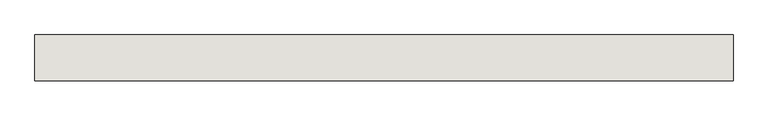
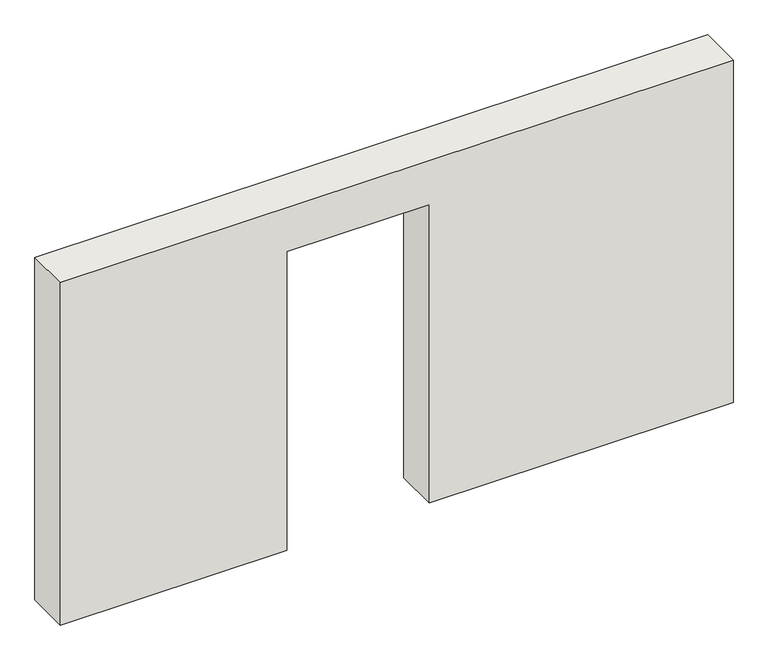
"""IFC4 building model written with IfcOpenShell, lengths in millimetres: wall geometry, 0_3d_modell."""

import ifcopenshell
import ifcopenshell.guid

model = None  # the IFC model being written
_history = None  # IfcOwnerHistory: only IFC2X3 demands one
_inside = {}  # id of a spatial element -> (the spatial element, [elements in it])
_under = {}  # id of a project, library or spatial element -> (it, [spatial elements below it])
_declared = {}  # id of a project -> (the project, [libraries it declares])
_typed = {}  # id of a type object -> (the type object, [elements of that type])
_made_of = {}  # id of a material, layer set ... -> (it, [elements and type objects made of it])


def new_model(schema):
    """Start an empty IFC model of exactly this schema.

    Asked for "IFC4X3", IfcOpenShell would pick the latest addendum, in which some entities
    have other attributes; the version numbers below select the first issue.
    IFC2X3 requires an IfcOwnerHistory on every rooted entity: one is made here for all.
    """
    global model, _history
    if schema == "IFC4X3":
        model = ifcopenshell.file(schema_version=(4, 3, 0, 0))
    else:
        model = ifcopenshell.file(schema=schema)
    _inside.clear()
    _under.clear()
    _declared.clear()
    _typed.clear()
    _made_of.clear()
    _history = None
    if model.schema == "IFC2X3":
        org = make("IfcOrganization", Name="unknown")
        user = make(
            "IfcPersonAndOrganization",
            ThePerson=make("IfcPerson", FamilyName="unknown"),
            TheOrganization=org,
        )
        app = make(
            "IfcApplication",
            ApplicationDeveloper=org,
            Version="unknown",
            ApplicationFullName="unknown",
            ApplicationIdentifier="unknown",
        )
        _history = make(
            "IfcOwnerHistory",
            OwningUser=user,
            OwningApplication=app,
            ChangeAction="ADDED",
            CreationDate=0,
        )
    return model


def make(cls, **values):
    """One entity of the class cls with the attributes given. An attribute that is None is left unset."""
    return model.create_entity(
        cls, **{name: value for name, value in values.items() if value is not None}
    )


def rooted(cls, **values):
    """An entity with a GlobalId (a new one), such as an element, a storey or a relation."""
    return make(cls, GlobalId=ifcopenshell.guid.new(), OwnerHistory=_history, **values)


def si_unit(unit_type, name, prefix=None):
    """IfcSIUnit, for example si_unit("LENGTHUNIT", "METRE", prefix="MILLI")."""
    return make("IfcSIUnit", UnitType=unit_type, Prefix=prefix, Name=name)


def assignment(units):
    """IfcUnitAssignment: the units of a project."""
    return None if units is None else make("IfcUnitAssignment", Units=units)


def point(xyz):
    """IfcCartesianPoint."""
    return None if xyz is None else make("IfcCartesianPoint", Coordinates=xyz)


def direction(xyz):
    """IfcDirection."""
    return None if xyz is None else make("IfcDirection", DirectionRatios=xyz)


def frame(location, z_axis=None, x_axis=None):
    """IfcAxis2Placement3D, a coordinate frame: its origin and axes. An axis left out is left unset."""
    return make(
        "IfcAxis2Placement3D",
        Location=point(location),
        Axis=direction(z_axis),
        RefDirection=direction(x_axis),
    )


def origin():
    """The frame at (0, 0, 0) with its axes left unset."""
    return frame((0.0, 0.0, 0.0))


def place(relative_to, where):
    """IfcLocalPlacement: puts the frame where relative to a parent placement (None: the world)."""
    return make(
        "IfcLocalPlacement", PlacementRelTo=relative_to, RelativePlacement=where
    )


def context(
    kind, dimensions, precision=None, world=None, true_north=None, identifier=None
):
    """IfcGeometricRepresentationContext, for example the 3D "Model" context."""
    return make(
        "IfcGeometricRepresentationContext",
        ContextIdentifier=identifier,
        ContextType=kind,
        CoordinateSpaceDimension=dimensions,
        Precision=precision,
        WorldCoordinateSystem=world,
        TrueNorth=true_north,
    )


def project(units=None, contexts=None):
    """IfcProject with its units and contexts."""
    return rooted(
        "IfcProject",
        Name="project",
        RepresentationContexts=contexts,
        UnitsInContext=assignment(units),
    )


def spatial(cls, under=None, at=None, **own):
    """A site, building, storey or space (cls), placed at a placement, below another one or the project."""
    s = rooted(cls, ObjectPlacement=at, **own)
    if under is not None:
        _under.setdefault(under.id(), (under, []))[1].append(s)
    return s


def polyline(points):
    """IfcPolyline through the points."""
    return make("IfcPolyline", Points=[point(p) for p in points])


def outline(outer, holes=None, kind="AREA"):
    """IfcArbitraryClosedProfileDef: a profile drawn as a closed curve; with holes, ...WithVoids."""
    if holes is None:
        return make("IfcArbitraryClosedProfileDef", ProfileType=kind, OuterCurve=outer)
    return make(
        "IfcArbitraryProfileDefWithVoids",
        ProfileType=kind,
        OuterCurve=outer,
        InnerCurves=holes,
    )


def extrude(swept, where, along, depth):
    """IfcExtrudedAreaSolid: the profile swept, set in the frame where, extruded along a direction by depth."""
    return make(
        "IfcExtrudedAreaSolid",
        SweptArea=swept,
        Position=where,
        ExtrudedDirection=direction(along),
        Depth=depth,
    )


def shape(context_of_items, identifier, shape_type, items):
    """IfcShapeRepresentation: the items that make up one representation, for example the "Body"."""
    return make(
        "IfcShapeRepresentation",
        ContextOfItems=context_of_items,
        RepresentationIdentifier=identifier,
        RepresentationType=shape_type,
        Items=items,
    )


def source(mapping_origin, context_of_items, identifier, shape_type, items):
    """IfcRepresentationMap: a shape defined once, which mapped items show again and again."""
    return make(
        "IfcRepresentationMap",
        MappingOrigin=mapping_origin,
        MappedRepresentation=shape(context_of_items, identifier, shape_type, items),
    )


def transform(
    local_origin,
    x_axis=None,
    y_axis=None,
    z_axis=None,
    scale=None,
    scale2=None,
    scale3=None,
    uniform=True,
):
    """IfcCartesianTransformationOperator3D, or its non-uniform kind. x_axis, y_axis, z_axis: its Axis1, 2, 3."""
    if uniform:
        return make(
            "IfcCartesianTransformationOperator3D",
            Axis1=direction(x_axis),
            Axis2=direction(y_axis),
            LocalOrigin=point(local_origin),
            Scale=scale,
            Axis3=direction(z_axis),
        )
    return make(
        "IfcCartesianTransformationOperator3DnonUniform",
        Axis1=direction(x_axis),
        Axis2=direction(y_axis),
        LocalOrigin=point(local_origin),
        Scale=scale,
        Axis3=direction(z_axis),
        Scale2=scale2,
        Scale3=scale3,
    )


def mapped(mapping_source, mapping_target):
    """IfcMappedItem: shows the shape of a source again, moved by a transform."""
    return make(
        "IfcMappedItem", MappingSource=mapping_source, MappingTarget=mapping_target
    )


def made_of(thing, what):
    """Note that an element or type object is made of a material, layer set ...; save() writes the relation."""
    if what is not None:
        _made_of.setdefault(what.id(), (what, []))[1].append(thing)
    return thing


def element(
    cls,
    number,
    at=None,
    inside=None,
    cuts=None,
    type_object=None,
    material=None,
    context=None,
    identifier="Body",
    shape_type=None,
    held_by="IfcProductDefinitionShape",
    body=None,
    shapes=None,
    **own,
):
    """One element of the class cls, such as IfcWall. Its Tag is "e" and its number.

    at: its placement. inside: the storey or other place that contains it. cuts: it is an
    opening in that element (IfcRelVoidsElement). A single representation is given by context,
    identifier, shape_type and body (its items); several are given by shapes. held_by: the class
    of the entity that holds the representations. save() writes the other relations.
    """
    e = rooted(cls, Tag="e%d" % number, ObjectPlacement=at, **own)
    if body is not None:
        shapes = [shape(context, identifier, shape_type, body)]
    if shapes is not None:
        e.Representation = make(held_by, Representations=shapes)
    if inside is not None:
        _inside.setdefault(inside.id(), (inside, []))[1].append(e)
    if cuts is not None:
        rooted(
            "IfcRelVoidsElement", RelatingBuildingElement=cuts, RelatedOpeningElement=e
        )
    if type_object is not None:
        _typed.setdefault(type_object.id(), (type_object, []))[1].append(e)
    return made_of(e, material)


def aggregate(whole, parts):
    """IfcRelAggregates: a whole, such as a stair, and the parts it consists of."""
    return rooted("IfcRelAggregates", RelatingObject=whole, RelatedObjects=parts)


def save(model, path):
    """Write the relations noted so far, then the file.

    IfcRelAggregates (storeys below a building ...), IfcRelContainedInSpatialStructure (elements
    in a storey), IfcRelDefinesByType, IfcRelAssociatesMaterial and IfcRelDeclares: one each for
    every whole, place, type object, material and project.
    """
    for whole, parts in _under.values():
        aggregate(whole, parts)
    for where, things in _inside.values():
        rooted(
            "IfcRelContainedInSpatialStructure",
            RelatedElements=things,
            RelatingStructure=where,
        )
    for kind, things in _typed.values():
        rooted("IfcRelDefinesByType", RelatedObjects=things, RelatingType=kind)
    for what, things in _made_of.values():
        rooted("IfcRelAssociatesMaterial", RelatedObjects=things, RelatingMaterial=what)
    for by, libraries in _declared.values():
        rooted("IfcRelDeclares", RelatingContext=by, RelatedDefinitions=libraries)
    model.write(path)


def wall_d88cb43b(model_context):
    return source(origin(), model_context, "Body", "SweptSolid", [
        extrude(outline(polyline([(2510.0, 2935.0), (0.0, 2935.0), (0.0, 5350.0), (2880.0, 5350.0), (2880.0, 0.0), (0.0, 0.0), (0.0, 1800.0), (2510.0, 1800.0), (2510.0, 2935.0)])), frame((0.0, 0.0, 0.0), z_axis=(0.0, 1.0, 0.0), x_axis=(0.0, 0.0, 1.0)), (0.0, 0.0, 1.0), 350.0),
    ])


if __name__ == "__main__":
    model = new_model("IFC4")
    model_context = context("Model", 3, world=origin())
    ifc_project = project(units=[si_unit("LENGTHUNIT", "METRE", prefix="MILLI")], contexts=[model_context])
    site = spatial("IfcSite", under=ifc_project)
    building = spatial("IfcBuilding", under=site)
    placement = place(None, origin())
    wall_shape = wall_d88cb43b(model_context)
    element("IfcWall", 1, ObjectType="0_3d_modell", at=placement, inside=building, context=model_context, shape_type="MappedRepresentation", body=[
        mapped(wall_shape, transform((0.0, 0.0, 0.0), x_axis=(1.0, 0.0, 0.0), y_axis=(0.0, 1.0, 0.0), z_axis=(0.0, 0.0, 1.0))),
    ])
    save(model, "model.ifc")

# Revit data of these elements
# Element 1 (IfcWall, "0_3d_modell")
#   Materials on its faces: "holzschalung"
# Materials
#   "holzschalung": class "Unassigned", colour RGB 128 128 128, transparency 0
